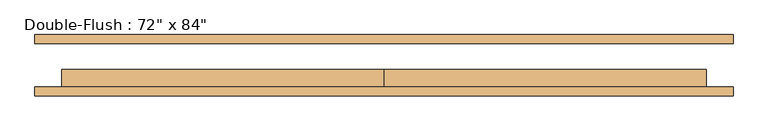
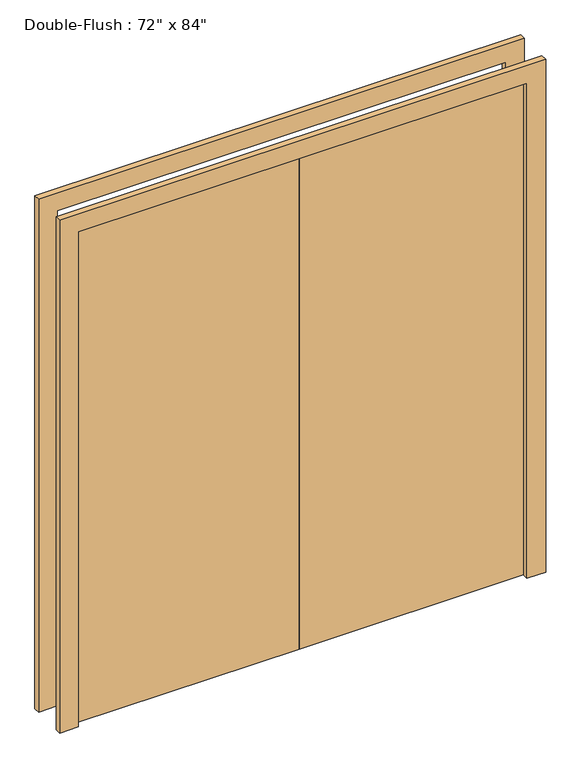
"""IFC4 building model written with IfcOpenShell, lengths in millimetres: door geometry."""

from ifc_helpers import new_model, si_unit, frame, origin, origin_with_axes, place, context, project, spatial, polyline, outline, extrude, source, transform, mapped, element, save


def door_e729474a(model_context):
    return source(origin(), model_context, "Body", "SweptSolid", [
        extrude(outline(polyline([(0.0, -61.9125), (0.0, -11.1125), (914.4, -11.1125), (914.4, -61.9125), (0.0, -61.9125)])), origin_with_axes(), (0.0, 0.0, 1.0), 2133.6),
        extrude(outline(polyline([(-914.4, -61.9125), (-914.4, -11.1125), (0.0, -11.1125), (0.0, -61.9125), (-914.4, -61.9125)])), origin_with_axes(), (0.0, 0.0, 1.0), 2133.6),
        extrude(outline(polyline([(2133.6, -914.4), (2133.6, 914.4), (0.0, 914.4), (0.0, 990.6), (2209.8, 990.6), (2209.8, -990.6), (0.0, -990.6), (0.0, -914.4), (2133.6, -914.4)])), frame((0.0, 61.9125, 0.0), z_axis=(0.0, 1.0, 0.0), x_axis=(0.0, 0.0, 1.0)), (0.0, 0.0, 1.0), 25.4),
        extrude(outline(polyline([(2133.6, -914.4), (2133.6, 914.4), (0.0, 914.4), (0.0, 990.6), (2209.8, 990.6), (2209.8, -990.6), (0.0, -990.6), (0.0, -914.4), (2133.6, -914.4)])), frame((0.0, -87.3125, 0.0), z_axis=(0.0, 1.0, 0.0), x_axis=(0.0, 0.0, 1.0)), (0.0, 0.0, 1.0), 25.4),
    ])


if __name__ == "__main__":
    model = new_model("IFC4")
    model_context = context("Model", 3, world=origin())
    ifc_project = project(units=[si_unit("LENGTHUNIT", "METRE", prefix="MILLI")], contexts=[model_context])
    site = spatial("IfcSite", under=ifc_project)
    building = spatial("IfcBuilding", under=site)
    placement = place(None, origin())
    door_shape = door_e729474a(model_context)
    element("IfcDoor", 1, ObjectType="Double-Flush : 72\" x 84\"", at=placement, inside=building, context=model_context, shape_type="MappedRepresentation", body=[
        mapped(door_shape, transform((0.0, 0.0, 0.0), x_axis=(1.0, 0.0, 0.0), y_axis=(0.0, 1.0, 0.0), z_axis=(0.0, 0.0, 1.0))),
    ])
    save(model, "model.ifc")

# Revit data of these elements
# Type "Double-Flush : 72\" x 84\""
#   Type Mark = "14"
#   Assembly Code = "C1020"
#   Thickness = 0' - 2"
#   Height = 7' - 0"
#   Trim Projection Ext = 0' - 1"
#   Trim Projection Int = 0' - 1"
#   Trim Width = 0' - 3"
#   Width = 6' - 0"
#   Door Material = Door - Panel
#   Frame Material = Door - Frame
#   Function = (empty or 0)
#   Wall Closure = (empty or 0)
# Element 1 (IfcDoor, "Double-Flush : 72\" x 84\"")
#   Materials on its faces: "Door - Frame", "Door - Panel"
# Materials
#   "Door - Panel": class "Wood", colour RGB 210 159 95, transparency 0
#   "Door - Frame": class "Miscellaneous", colour RGB 118 70 51, transparency 0
